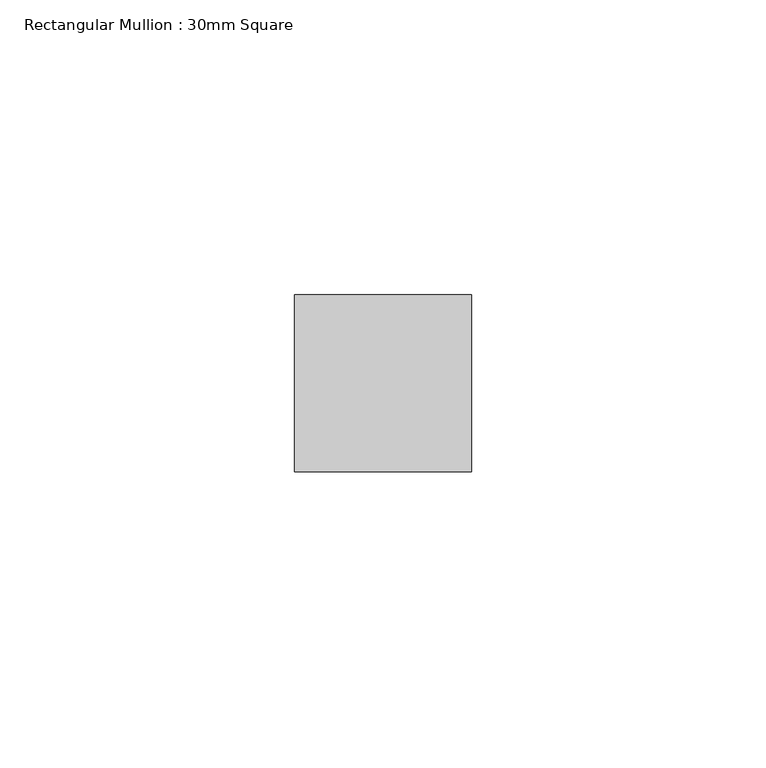
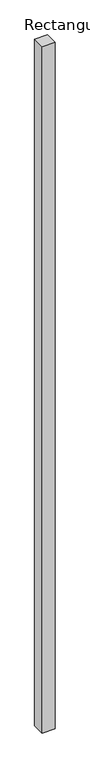
"""IFC4 building model written with IfcOpenShell, lengths in millimetres: member geometry, Rectangular Mullion : 30mm Square."""

from ifc_helpers import new_model, si_unit, frame, origin, place, context, project, spatial, polyline, outline, extrude, source, transform, mapped, element, save


def rectangular_mullion_30mm_square_54935cf5(model_context):
    return source(origin(), model_context, "Body", "SweptSolid", [
        extrude(outline(polyline([(15.0, 15.0), (15.0, -15.0), (-15.0, -15.0), (-15.0, 15.0), (15.0, 15.0)])), frame((0.0, 0.0, -1688.5217616), z_axis=(0.0, 0.0, 1.0), x_axis=(1.0, 0.0, 0.0)), (0.0, 0.0, 1.0), 1688.5217616),
    ])


if __name__ == "__main__":
    model = new_model("IFC4")
    model_context = context("Model", 3, world=origin())
    ifc_project = project(units=[si_unit("LENGTHUNIT", "METRE", prefix="MILLI")], contexts=[model_context])
    site = spatial("IfcSite", under=ifc_project)
    building = spatial("IfcBuilding", under=site)
    placement = place(None, origin())
    rectangular_mullion_30mm_square_shape = rectangular_mullion_30mm_square_54935cf5(model_context)
    element("IfcMember", 1, ObjectType="Rectangular Mullion : 30mm Square", at=placement, inside=building, context=model_context, shape_type="MappedRepresentation", body=[
        mapped(rectangular_mullion_30mm_square_shape, transform((0.0, 0.0, 0.0), x_axis=(1.0, 0.0, 0.0), y_axis=(0.0, 1.0, 0.0), z_axis=(0.0, 0.0, 1.0))),
    ])
    save(model, "model.ifc")

# Revit data of these elements
# Type "Rectangular Mullion : 30mm Square"
#   built-in parameter 1007304 = 0.0984252 (stored number, unit not read)
#   built-in parameter 1007301 = 0.0492126 (stored number, unit not read)
#   built-in parameter 1007300 = 0.0492126 (stored number, unit not read)
# Element 1 (IfcMember, "Rectangular Mullion : 30mm Square")
#   Materials on its faces: "Aluminum"
# Materials
#   "Aluminum": class "Metal", colour RGB 244 244 244, transparency 0, Description = "Aluminum 6061", Cost = 0
